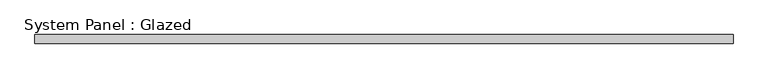
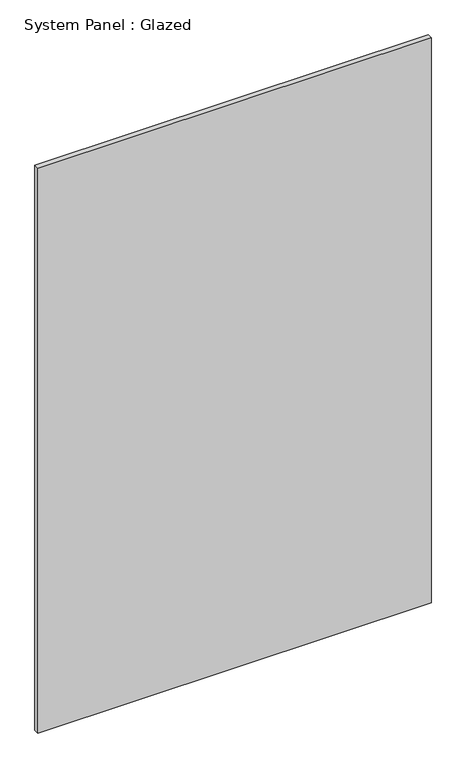
"""IFC4 building model written with IfcOpenShell, lengths in millimetres: plate geometry, System Panel : Glazed."""

from ifc_helpers import new_model, si_unit, origin, origin_with_axes, place, context, project, spatial, polyline, outline, extrude, source, transform, mapped, element, save


def system_panel_glazed_156c2b36(model_context):
    return source(origin(), model_context, "Body", "SweptSolid", [
        extrude(outline(polyline([(962.5000001, 24.5), (-962.5000001, 24.5), (-962.5000001, 49.5), (962.5000001, 49.5), (962.5000001, 24.5)])), origin_with_axes(), (0.0, 0.0, 1.0), 2925.0),
    ])


if __name__ == "__main__":
    model = new_model("IFC4")
    model_context = context("Model", 3, world=origin())
    ifc_project = project(units=[si_unit("LENGTHUNIT", "METRE", prefix="MILLI")], contexts=[model_context])
    site = spatial("IfcSite", under=ifc_project)
    building = spatial("IfcBuilding", under=site)
    placement = place(None, origin())
    system_panel_glazed_shape = system_panel_glazed_156c2b36(model_context)
    element("IfcPlate", 1, ObjectType="System Panel : Glazed", at=placement, inside=building, context=model_context, shape_type="MappedRepresentation", body=[
        mapped(system_panel_glazed_shape, transform((0.0, 0.0, 0.0), x_axis=(1.0, 0.0, 0.0), y_axis=(0.0, 1.0, 0.0), z_axis=(0.0, 0.0, 1.0))),
    ])
    save(model, "model.ifc")

# Revit data of these elements
# Element 1 (IfcPlate, "System Panel : Glazed")
#   Materials on its faces: "Glass"
# Materials
#   "Glass": class "Glass", colour RGB 0 128 192, transparency 0.9
